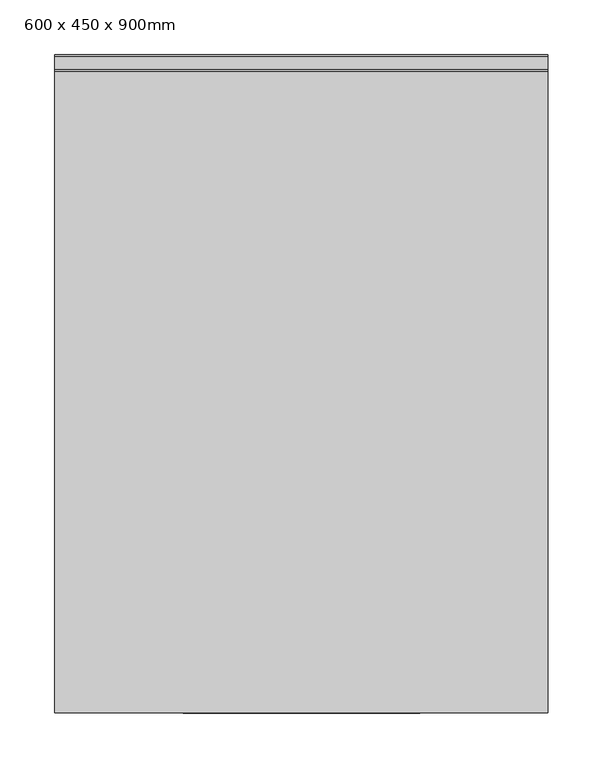
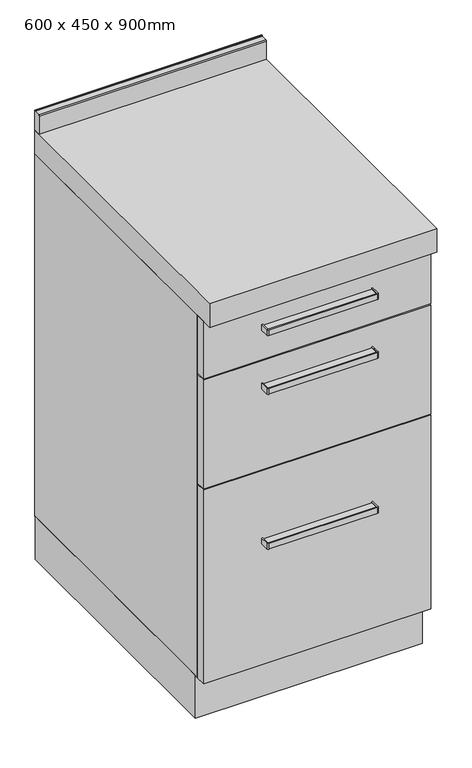
"""IFC4 building model written with IfcOpenShell, lengths in millimetres: furniture geometry, Küchenelement (1) - 2 Schubläden : 600 x 450 x 900mm."""

from ifc_helpers import new_model, si_unit, point, frame, frame_2d, origin, origin_with_axes, place, context, project, spatial, polyline, circle_curve, trimmed, segment, composite_curve, outline, extrude, source, transform, mapped, element, save


def furniture_600_x_450_x_900mm_2347578c(model_context):
    return source(origin(), model_context, "Body", "SweptSolid", [
        extrude(outline(composite_curve([segment(polyline([(-63.2996736, -577.0), (152.7003264, -577.0), (152.7003264, -597.5)]), True, "CONTINUOUS"), segment(trimmed(circle_curve(frame_2d((152.2003264, -597.5)), 0.5), [point((152.7003264, -597.5))], [point((152.2003264, -598.0))], False, "CARTESIAN"), True, "CONTINUOUS"), segment(polyline([(152.2003264, -598.0), (-62.7996736, -598.0)]), True, "CONTINUOUS"), segment(trimmed(circle_curve(frame_2d((-62.7996736, -597.5)), 0.5), [point((-62.7996736, -598.0))], [point((-63.2996736, -597.5))], False, "CARTESIAN"), True, "CONTINUOUS"), segment(polyline([(-63.2996736, -597.5), (-63.2996736, -577.0)]), True, "CONTINUOUS")], self_intersect=False)), frame((0.0, 0.0, 346.445389), z_axis=(0.0, 0.0, 1.0), x_axis=(1.0, 0.0, 0.0)), (0.0, 0.0, 1.0), 6.4890959),
        extrude(outline(composite_curve([segment(polyline([(-65.2996736, -577.0), (-63.2996736, -577.0), (-63.2996736, -597.5)]), True, "CONTINUOUS"), segment(trimmed(circle_curve(frame_2d((-62.7996736, -597.5)), 0.5), [point((-63.2996736, -597.5))], [point((-62.7996736, -598.0))], True, "CARTESIAN"), True, "CONTINUOUS"), segment(polyline([(-62.7996736, -598.0), (152.2003264, -598.0)]), True, "CONTINUOUS"), segment(trimmed(circle_curve(frame_2d((152.2003264, -597.5)), 0.5), [point((152.2003264, -598.0))], [point((152.7003264, -597.5))], True, "CARTESIAN"), True, "CONTINUOUS"), segment(polyline([(152.7003264, -597.5), (152.7003264, -577.0), (154.7003264, -577.0), (154.7003264, -597.5)]), True, "CONTINUOUS"), segment(trimmed(circle_curve(frame_2d((152.2003264, -597.5)), 2.5), [point((154.7003264, -597.5))], [point((152.2003264, -600.0))], False, "CARTESIAN"), True, "CONTINUOUS"), segment(polyline([(152.2003264, -600.0), (-62.7996736, -600.0)]), True, "CONTINUOUS"), segment(trimmed(circle_curve(frame_2d((-62.7996736, -597.5)), 2.5), [point((-62.7996736, -600.0))], [point((-65.2996736, -597.5))], False, "CARTESIAN"), True, "CONTINUOUS"), segment(polyline([(-65.2996736, -597.5), (-65.2996736, -577.0)]), True, "CONTINUOUS")], self_intersect=False)), frame((0.0, 0.0, 343.68), z_axis=(0.0, 0.0, 1.0), x_axis=(1.0, 0.0, 0.0)), (0.0, 0.0, 1.0), 12.0),
        extrude(outline(composite_curve([segment(polyline([(-63.2996736, -577.0), (152.7003264, -577.0), (152.7003264, -597.5)]), True, "CONTINUOUS"), segment(trimmed(circle_curve(frame_2d((152.2003264, -597.5)), 0.5), [point((152.7003264, -597.5))], [point((152.2003264, -598.0))], False, "CARTESIAN"), True, "CONTINUOUS"), segment(polyline([(152.2003264, -598.0), (-62.7996736, -598.0)]), True, "CONTINUOUS"), segment(trimmed(circle_curve(frame_2d((-62.7996736, -597.5)), 0.5), [point((-62.7996736, -598.0))], [point((-63.2996736, -597.5))], False, "CARTESIAN"), True, "CONTINUOUS"), segment(polyline([(-63.2996736, -597.5), (-63.2996736, -577.0)]), True, "CONTINUOUS")], self_intersect=False)), frame((0.0, 0.0, 671.435389), z_axis=(0.0, 0.0, 1.0), x_axis=(1.0, 0.0, 0.0)), (0.0, 0.0, 1.0), 6.4890959),
        extrude(outline(composite_curve([segment(polyline([(-65.2996736, -577.0), (-63.2996736, -577.0), (-63.2996736, -597.5)]), True, "CONTINUOUS"), segment(trimmed(circle_curve(frame_2d((-62.7996736, -597.5)), 0.5), [point((-63.2996736, -597.5))], [point((-62.7996736, -598.0))], True, "CARTESIAN"), True, "CONTINUOUS"), segment(polyline([(-62.7996736, -598.0), (152.2003264, -598.0)]), True, "CONTINUOUS"), segment(trimmed(circle_curve(frame_2d((152.2003264, -597.5)), 0.5), [point((152.2003264, -598.0))], [point((152.7003264, -597.5))], True, "CARTESIAN"), True, "CONTINUOUS"), segment(polyline([(152.7003264, -597.5), (152.7003264, -577.0), (154.7003264, -577.0), (154.7003264, -597.5)]), True, "CONTINUOUS"), segment(trimmed(circle_curve(frame_2d((152.2003264, -597.5)), 2.5), [point((154.7003264, -597.5))], [point((152.2003264, -600.0))], False, "CARTESIAN"), True, "CONTINUOUS"), segment(polyline([(152.2003264, -600.0), (-62.7996736, -600.0)]), True, "CONTINUOUS"), segment(trimmed(circle_curve(frame_2d((-62.7996736, -597.5)), 2.5), [point((-62.7996736, -600.0))], [point((-65.2996736, -597.5))], False, "CARTESIAN"), True, "CONTINUOUS"), segment(polyline([(-65.2996736, -597.5), (-65.2996736, -577.0)]), True, "CONTINUOUS")], self_intersect=False)), frame((0.0, 0.0, 668.67), z_axis=(0.0, 0.0, 1.0), x_axis=(1.0, 0.0, 0.0)), (0.0, 0.0, 1.0), 12.0),
        extrude(outline(composite_curve([segment(polyline([(-63.2996736, -577.0), (152.7003264, -577.0), (152.7003264, -597.5)]), True, "CONTINUOUS"), segment(trimmed(circle_curve(frame_2d((152.2003264, -597.5)), 0.5), [point((152.7003264, -597.5))], [point((152.2003264, -598.0))], False, "CARTESIAN"), True, "CONTINUOUS"), segment(polyline([(152.2003264, -598.0), (-62.7996736, -598.0)]), True, "CONTINUOUS"), segment(trimmed(circle_curve(frame_2d((-62.7996736, -597.5)), 0.5), [point((-62.7996736, -598.0))], [point((-63.2996736, -597.5))], False, "CARTESIAN"), True, "CONTINUOUS"), segment(polyline([(-63.2996736, -597.5), (-63.2996736, -577.0)]), True, "CONTINUOUS")], self_intersect=False)), frame((0.0, 0.0, 794.465389), z_axis=(0.0, 0.0, 1.0), x_axis=(1.0, 0.0, 0.0)), (0.0, 0.0, 1.0), 6.4890959),
        extrude(outline(composite_curve([segment(polyline([(-65.2996736, -577.0), (-63.2996736, -577.0), (-63.2996736, -597.5)]), True, "CONTINUOUS"), segment(trimmed(circle_curve(frame_2d((-62.7996736, -597.5)), 0.5), [point((-63.2996736, -597.5))], [point((-62.7996736, -598.0))], True, "CARTESIAN"), True, "CONTINUOUS"), segment(polyline([(-62.7996736, -598.0), (152.2003264, -598.0)]), True, "CONTINUOUS"), segment(trimmed(circle_curve(frame_2d((152.2003264, -597.5)), 0.5), [point((152.2003264, -598.0))], [point((152.7003264, -597.5))], True, "CARTESIAN"), True, "CONTINUOUS"), segment(polyline([(152.7003264, -597.5), (152.7003264, -577.0), (154.7003264, -577.0), (154.7003264, -597.5)]), True, "CONTINUOUS"), segment(trimmed(circle_curve(frame_2d((152.2003264, -597.5)), 2.5), [point((154.7003264, -597.5))], [point((152.2003264, -600.0))], False, "CARTESIAN"), True, "CONTINUOUS"), segment(polyline([(152.2003264, -600.0), (-62.7996736, -600.0)]), True, "CONTINUOUS"), segment(trimmed(circle_curve(frame_2d((-62.7996736, -597.5)), 2.5), [point((-62.7996736, -600.0))], [point((-65.2996736, -597.5))], False, "CARTESIAN"), True, "CONTINUOUS"), segment(polyline([(-65.2996736, -597.5), (-65.2996736, -577.0)]), True, "CONTINUOUS")], self_intersect=False)), frame((0.0, 0.0, 791.7), z_axis=(0.0, 0.0, 1.0), x_axis=(1.0, 0.0, 0.0)), (0.0, 0.0, 1.0), 12.0),
        extrude(outline(polyline([(269.7003264, -580.0), (-180.2996736, -580.0), (-180.2996736, -558.0), (269.7003264, -558.0), (269.7003264, -580.0)])), frame((0.0, 0.0, 730.0), z_axis=(0.0, 0.0, 1.0), x_axis=(1.0, 0.0, 0.0)), (0.0, 0.0, 1.0), 120.0),
        extrude(outline(polyline([(269.7003264, -580.0), (-180.2996736, -580.0), (-180.2996736, -558.0), (269.7003264, -558.0), (269.7003264, -580.0)])), frame((0.0, 0.0, 498.5), z_axis=(0.0, 0.0, 1.0), x_axis=(1.0, 0.0, 0.0)), (0.0, 0.0, 1.0), 228.5),
        extrude(outline(polyline([(269.7003264, -580.0), (-180.2996736, -580.0), (-180.2996736, -558.0), (269.7003264, -558.0), (269.7003264, -580.0)])), frame((0.0, 0.0, 90.0), z_axis=(0.0, 0.0, 1.0), x_axis=(1.0, 0.0, 0.0)), (0.0, 0.0, 1.0), 406.5),
        extrude(outline(composite_curve([segment(polyline([(0.0, 942.0034681), (0.0, 900.0), (-15.0, 900.0), (-15.0, 938.0)]), True, "CONTINUOUS"), segment(trimmed(circle_curve(frame_2d((-13.0, 938.0)), 2.0), [point((-15.0, 938.0))], [point((-13.0, 940.0))], False, "CARTESIAN"), True, "CONTINUOUS"), segment(polyline([(-13.0, 940.0), (-1.50449, 940.0), (-1.50449, 942.0034681), (0.0, 942.0034681)]), True, "CONTINUOUS")], self_intersect=False)), frame((-180.2996736, 0.0, 0.0), z_axis=(1.0, 0.0, 0.0), x_axis=(0.0, 1.0, 0.0)), (0.0, 0.0, 1.0), 450.0),
        extrude(outline(polyline([(269.7003264, -0.533703), (269.7003264, -550.533703), (-180.2996736, -550.533703), (-180.2996736, -0.533703), (269.7003264, -0.533703)])), origin_with_axes(), (0.0, 0.0, 1.0), 90.0),
        extrude(outline(polyline([(269.7003264, 0.0), (269.7003264, -600.0), (-180.2996736, -600.0), (-180.2996736, 0.0), (269.7003264, 0.0)])), frame((0.0, 0.0, 850.0), z_axis=(0.0, 0.0, 1.0), x_axis=(1.0, 0.0, 0.0)), (0.0, 0.0, 1.0), 50.0),
        extrude(outline(polyline([(269.7003264, 0.0), (269.7003264, -558.0), (247.7003264, -558.0), (247.7003264, -22.0), (-158.2996736, -22.0), (-158.2996736, -558.0), (-180.2996736, -558.0), (-180.2996736, 0.0), (269.7003264, 0.0)])), frame((0.0, 0.0, 90.0), z_axis=(0.0, 0.0, 1.0), x_axis=(1.0, 0.0, 0.0)), (0.0, 0.0, 1.0), 760.0),
    ])


if __name__ == "__main__":
    model = new_model("IFC4")
    model_context = context("Model", 3, world=origin())
    ifc_project = project(units=[si_unit("LENGTHUNIT", "METRE", prefix="MILLI")], contexts=[model_context])
    site = spatial("IfcSite", under=ifc_project)
    building = spatial("IfcBuilding", under=site)
    placement = place(None, origin())
    furniture_600_x_450_x_900mm_shape = furniture_600_x_450_x_900mm_2347578c(model_context)
    element("IfcFurniture", 1, ObjectType="Küchenelement (1) - 2 Schubläden : 600 x 450 x 900mm", at=placement, inside=building, context=model_context, shape_type="MappedRepresentation", body=[
        mapped(furniture_600_x_450_x_900mm_shape, transform((0.0, 0.0, 0.0), x_axis=(1.0, 0.0, 0.0), y_axis=(0.0, 1.0, 0.0), z_axis=(0.0, 0.0, 1.0))),
    ])
    save(model, "model.ifc")

# Revit data of these elements
# Type "Küchenelement (1) - 2 Schubläden : 600 x 450 x 900mm"
#   Assembly Code = "C1030400"
#   Länge 3 = 0.12303 m
#   Länge 2 = 0.32499 m
#   Länge 1 = 0.35568 m
#   Depth = 0.600 m
#   Height = 0.900 m
#   Width = 0.450 m
#   1 = 0.000 m
#   Obermaterial = none
#   Material = none
#   Griffmaterial = none
# Element 1 (IfcFurniture, "Küchenelement (1) - 2 Schubläden : 600 x 450 x 900mm")
#   Materials on its faces: "Holz - Birke"
# Materials
#   "Holz - Birke": class "Holz", colour RGB 213 164 103, transparency 0, Cost = 0
